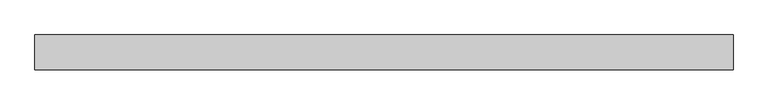
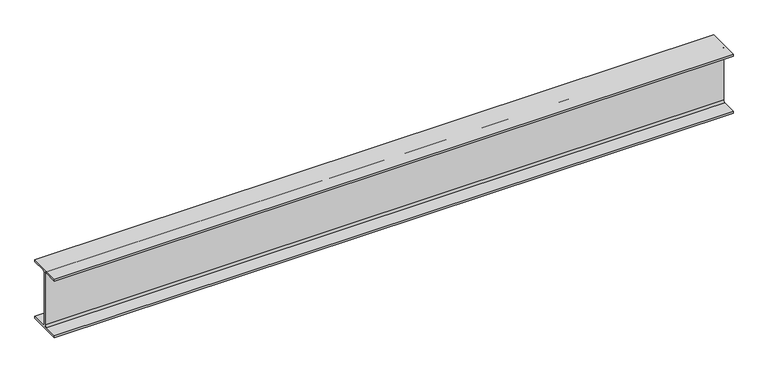
"""IFC4 building model written with IfcOpenShell, lengths in millimetres: beam geometry, Old_Steel Beam_H-KSD3502 : H_SB_ASB_H-200×200x8x12."""

import ifcopenshell
import ifcopenshell.guid

model = None  # the IFC model being written
_history = None  # IfcOwnerHistory: only IFC2X3 demands one
_inside = {}  # id of a spatial element -> (the spatial element, [elements in it])
_under = {}  # id of a project, library or spatial element -> (it, [spatial elements below it])
_declared = {}  # id of a project -> (the project, [libraries it declares])
_typed = {}  # id of a type object -> (the type object, [elements of that type])
_made_of = {}  # id of a material, layer set ... -> (it, [elements and type objects made of it])


def new_model(schema):
    """Start an empty IFC model of exactly this schema.

    Asked for "IFC4X3", IfcOpenShell would pick the latest addendum, in which some entities
    have other attributes; the version numbers below select the first issue.
    IFC2X3 requires an IfcOwnerHistory on every rooted entity: one is made here for all.
    """
    global model, _history
    if schema == "IFC4X3":
        model = ifcopenshell.file(schema_version=(4, 3, 0, 0))
    else:
        model = ifcopenshell.file(schema=schema)
    _inside.clear()
    _under.clear()
    _declared.clear()
    _typed.clear()
    _made_of.clear()
    _history = None
    if model.schema == "IFC2X3":
        org = make("IfcOrganization", Name="unknown")
        user = make(
            "IfcPersonAndOrganization",
            ThePerson=make("IfcPerson", FamilyName="unknown"),
            TheOrganization=org,
        )
        app = make(
            "IfcApplication",
            ApplicationDeveloper=org,
            Version="unknown",
            ApplicationFullName="unknown",
            ApplicationIdentifier="unknown",
        )
        _history = make(
            "IfcOwnerHistory",
            OwningUser=user,
            OwningApplication=app,
            ChangeAction="ADDED",
            CreationDate=0,
        )
    return model


def make(cls, **values):
    """One entity of the class cls with the attributes given. An attribute that is None is left unset."""
    return model.create_entity(
        cls, **{name: value for name, value in values.items() if value is not None}
    )


def rooted(cls, **values):
    """An entity with a GlobalId (a new one), such as an element, a storey or a relation."""
    return make(cls, GlobalId=ifcopenshell.guid.new(), OwnerHistory=_history, **values)


def si_unit(unit_type, name, prefix=None):
    """IfcSIUnit, for example si_unit("LENGTHUNIT", "METRE", prefix="MILLI")."""
    return make("IfcSIUnit", UnitType=unit_type, Prefix=prefix, Name=name)


def assignment(units):
    """IfcUnitAssignment: the units of a project."""
    return None if units is None else make("IfcUnitAssignment", Units=units)


def point(xyz):
    """IfcCartesianPoint."""
    return None if xyz is None else make("IfcCartesianPoint", Coordinates=xyz)


def direction(xyz):
    """IfcDirection."""
    return None if xyz is None else make("IfcDirection", DirectionRatios=xyz)


def frame(location, z_axis=None, x_axis=None):
    """IfcAxis2Placement3D, a coordinate frame: its origin and axes. An axis left out is left unset."""
    return make(
        "IfcAxis2Placement3D",
        Location=point(location),
        Axis=direction(z_axis),
        RefDirection=direction(x_axis),
    )


def frame_2d(location, x_axis=None):
    """IfcAxis2Placement2D, a coordinate frame in the plane: its origin and x axis."""
    return make(
        "IfcAxis2Placement2D", Location=point(location), RefDirection=direction(x_axis)
    )


def origin():
    """The frame at (0, 0, 0) with its axes left unset."""
    return frame((0.0, 0.0, 0.0))


def place(relative_to, where):
    """IfcLocalPlacement: puts the frame where relative to a parent placement (None: the world)."""
    return make(
        "IfcLocalPlacement", PlacementRelTo=relative_to, RelativePlacement=where
    )


def context(
    kind, dimensions, precision=None, world=None, true_north=None, identifier=None
):
    """IfcGeometricRepresentationContext, for example the 3D "Model" context."""
    return make(
        "IfcGeometricRepresentationContext",
        ContextIdentifier=identifier,
        ContextType=kind,
        CoordinateSpaceDimension=dimensions,
        Precision=precision,
        WorldCoordinateSystem=world,
        TrueNorth=true_north,
    )


def project(units=None, contexts=None):
    """IfcProject with its units and contexts."""
    return rooted(
        "IfcProject",
        Name="project",
        RepresentationContexts=contexts,
        UnitsInContext=assignment(units),
    )


def spatial(cls, under=None, at=None, **own):
    """A site, building, storey or space (cls), placed at a placement, below another one or the project."""
    s = rooted(cls, ObjectPlacement=at, **own)
    if under is not None:
        _under.setdefault(under.id(), (under, []))[1].append(s)
    return s


def polyline(points):
    """IfcPolyline through the points."""
    return make("IfcPolyline", Points=[point(p) for p in points])


def circle_curve(where, radius):
    """IfcCircle in the frame where."""
    return make("IfcCircle", Position=where, Radius=radius)


def trimmed(basis, trim1, trim2, sense, master):
    """IfcTrimmedCurve: the piece of a basis curve between two trims."""
    return make(
        "IfcTrimmedCurve",
        BasisCurve=basis,
        Trim1=trim1,
        Trim2=trim2,
        SenseAgreement=sense,
        MasterRepresentation=master,
    )


def segment(curve, same_sense, transition):
    """IfcCompositeCurveSegment."""
    return make(
        "IfcCompositeCurveSegment",
        Transition=transition,
        SameSense=same_sense,
        ParentCurve=curve,
    )


def composite_curve(segments, self_intersect=None):
    """IfcCompositeCurve: segments joined end to end."""
    return make("IfcCompositeCurve", Segments=segments, SelfIntersect=self_intersect)


def outline(outer, holes=None, kind="AREA"):
    """IfcArbitraryClosedProfileDef: a profile drawn as a closed curve; with holes, ...WithVoids."""
    if holes is None:
        return make("IfcArbitraryClosedProfileDef", ProfileType=kind, OuterCurve=outer)
    return make(
        "IfcArbitraryProfileDefWithVoids",
        ProfileType=kind,
        OuterCurve=outer,
        InnerCurves=holes,
    )


def extrude(swept, where, along, depth):
    """IfcExtrudedAreaSolid: the profile swept, set in the frame where, extruded along a direction by depth."""
    return make(
        "IfcExtrudedAreaSolid",
        SweptArea=swept,
        Position=where,
        ExtrudedDirection=direction(along),
        Depth=depth,
    )


def shape(context_of_items, identifier, shape_type, items):
    """IfcShapeRepresentation: the items that make up one representation, for example the "Body"."""
    return make(
        "IfcShapeRepresentation",
        ContextOfItems=context_of_items,
        RepresentationIdentifier=identifier,
        RepresentationType=shape_type,
        Items=items,
    )


def source(mapping_origin, context_of_items, identifier, shape_type, items):
    """IfcRepresentationMap: a shape defined once, which mapped items show again and again."""
    return make(
        "IfcRepresentationMap",
        MappingOrigin=mapping_origin,
        MappedRepresentation=shape(context_of_items, identifier, shape_type, items),
    )


def transform(
    local_origin,
    x_axis=None,
    y_axis=None,
    z_axis=None,
    scale=None,
    scale2=None,
    scale3=None,
    uniform=True,
):
    """IfcCartesianTransformationOperator3D, or its non-uniform kind. x_axis, y_axis, z_axis: its Axis1, 2, 3."""
    if uniform:
        return make(
            "IfcCartesianTransformationOperator3D",
            Axis1=direction(x_axis),
            Axis2=direction(y_axis),
            LocalOrigin=point(local_origin),
            Scale=scale,
            Axis3=direction(z_axis),
        )
    return make(
        "IfcCartesianTransformationOperator3DnonUniform",
        Axis1=direction(x_axis),
        Axis2=direction(y_axis),
        LocalOrigin=point(local_origin),
        Scale=scale,
        Axis3=direction(z_axis),
        Scale2=scale2,
        Scale3=scale3,
    )


def mapped(mapping_source, mapping_target):
    """IfcMappedItem: shows the shape of a source again, moved by a transform."""
    return make(
        "IfcMappedItem", MappingSource=mapping_source, MappingTarget=mapping_target
    )


def made_of(thing, what):
    """Note that an element or type object is made of a material, layer set ...; save() writes the relation."""
    if what is not None:
        _made_of.setdefault(what.id(), (what, []))[1].append(thing)
    return thing


def element(
    cls,
    number,
    at=None,
    inside=None,
    cuts=None,
    type_object=None,
    material=None,
    context=None,
    identifier="Body",
    shape_type=None,
    held_by="IfcProductDefinitionShape",
    body=None,
    shapes=None,
    **own,
):
    """One element of the class cls, such as IfcWall. Its Tag is "e" and its number.

    at: its placement. inside: the storey or other place that contains it. cuts: it is an
    opening in that element (IfcRelVoidsElement). A single representation is given by context,
    identifier, shape_type and body (its items); several are given by shapes. held_by: the class
    of the entity that holds the representations. save() writes the other relations.
    """
    e = rooted(cls, Tag="e%d" % number, ObjectPlacement=at, **own)
    if body is not None:
        shapes = [shape(context, identifier, shape_type, body)]
    if shapes is not None:
        e.Representation = make(held_by, Representations=shapes)
    if inside is not None:
        _inside.setdefault(inside.id(), (inside, []))[1].append(e)
    if cuts is not None:
        rooted(
            "IfcRelVoidsElement", RelatingBuildingElement=cuts, RelatedOpeningElement=e
        )
    if type_object is not None:
        _typed.setdefault(type_object.id(), (type_object, []))[1].append(e)
    return made_of(e, material)


def aggregate(whole, parts):
    """IfcRelAggregates: a whole, such as a stair, and the parts it consists of."""
    return rooted("IfcRelAggregates", RelatingObject=whole, RelatedObjects=parts)


def save(model, path):
    """Write the relations noted so far, then the file.

    IfcRelAggregates (storeys below a building ...), IfcRelContainedInSpatialStructure (elements
    in a storey), IfcRelDefinesByType, IfcRelAssociatesMaterial and IfcRelDeclares: one each for
    every whole, place, type object, material and project.
    """
    for whole, parts in _under.values():
        aggregate(whole, parts)
    for where, things in _inside.values():
        rooted(
            "IfcRelContainedInSpatialStructure",
            RelatedElements=things,
            RelatingStructure=where,
        )
    for kind, things in _typed.values():
        rooted("IfcRelDefinesByType", RelatedObjects=things, RelatingType=kind)
    for what, things in _made_of.values():
        rooted("IfcRelAssociatesMaterial", RelatedObjects=things, RelatingMaterial=what)
    for by, libraries in _declared.values():
        rooted("IfcRelDeclares", RelatingContext=by, RelatedDefinitions=libraries)
    model.write(path)


def beam_5e19d841(model_context):
    return source(origin(), model_context, "Body", "SweptSolid", [
        extrude(outline(composite_curve([segment(polyline([(82.5, -141.5), (82.5, -151.7), (-82.5, -151.7), (-82.5, -141.5), (-11.9, -141.5)]), True, "CONTINUOUS"), segment(trimmed(circle_curve(frame_2d((-11.9, -132.6)), 8.9), [point((-11.9, -141.5))], [point((-3.0, -132.6))], True, "CARTESIAN"), True, "CONTINUOUS"), segment(polyline([(-3.0, -132.6), (-3.0, 132.6)]), True, "CONTINUOUS"), segment(trimmed(circle_curve(frame_2d((-11.9, 132.6)), 8.9), [point((-3.0, 132.6))], [point((-11.9, 141.5))], True, "CARTESIAN"), True, "CONTINUOUS"), segment(polyline([(-11.9, 141.5), (-82.5, 141.5), (-82.5, 151.7), (82.5, 151.7), (82.5, 141.5), (11.9, 141.5)]), True, "CONTINUOUS"), segment(trimmed(circle_curve(frame_2d((11.9, 132.6)), 8.9), [point((11.9, 141.5))], [point((3.0, 132.6))], True, "CARTESIAN"), True, "CONTINUOUS"), segment(polyline([(3.0, 132.6), (3.0, -132.6)]), True, "CONTINUOUS"), segment(trimmed(circle_curve(frame_2d((11.9, -132.6)), 8.9), [point((3.0, -132.6))], [point((11.9, -141.5))], True, "CARTESIAN"), True, "CONTINUOUS"), segment(polyline([(11.9, -141.5), (82.5, -141.5)]), True, "CONTINUOUS")], self_intersect=False)), frame((-1721.7329802, 0.0, 0.0), z_axis=(1.0, 0.0, 0.0), x_axis=(0.0, 1.0, 0.0)), (0.0, 0.0, 1.0), 3316.0486402),
    ])


if __name__ == "__main__":
    model = new_model("IFC4")
    model_context = context("Model", 3, world=origin())
    ifc_project = project(units=[si_unit("LENGTHUNIT", "METRE", prefix="MILLI")], contexts=[model_context])
    site = spatial("IfcSite", under=ifc_project)
    building = spatial("IfcBuilding", under=site)
    placement = place(None, origin())
    beam_shape = beam_5e19d841(model_context)
    element("IfcBeam", 1, ObjectType="Old_Steel Beam_H-KSD3502 : H_SB_ASB_H-200×200x8x12", at=placement, inside=building, context=model_context, shape_type="MappedRepresentation", body=[
        mapped(beam_shape, transform((0.0, 0.0, 0.0), x_axis=(1.0, 0.0, 0.0), y_axis=(0.0, 1.0, 0.0), z_axis=(0.0, 0.0, 1.0))),
    ])
    save(model, "model.ifc")

# Revit data of these elements
# Type "Old_Steel Beam_H-KSD3502 : H_SB_ASB_H-200×200x8x12"
#   Width = 20.0 cm
#   Web Thickness = 0.8 cm
#   Web Fillet = 1.3 cm
#   Warping Constant = 141376.0 cm⁶
#   Torsional Moment of Inertia = 26.2485 cm⁴
#   Torsional Modulus = 1.0 cm³
#   Section Area = 63.53 cm²
#   Plastic Modulus weak axis = 244.0 cm³
#   Plastic Modulus strong axis = 525.0 cm³
#   Perimeter = 1.16 m²/m
#   Nominal Weight = 49.90 kgf/m
#   Moment of Inertia weak axis = 1600.00 cm⁴
#   Moment of Inertia strong axis = 4720.00 cm⁴
#   Height = 20.0 cm
#   Flange Thickness = 1.2 cm
#   Elastic Modulus weak axis = 160.0 cm³
#   Elastic Modulus strong axis = 472.0 cm³
#   Centroid Vertical = 10.0 cm
#   Centroid Horizontal = 10.0 cm
#   Length [instance default] = 1.5240 m
#   Structural Material [instance default] = Steel, 45-345
#   Assembly Code = ""
# Element 1 (IfcBeam, "Old_Steel Beam_H-KSD3502 : H_SB_ASB_H-200×200x8x12")
#   Structural Material = none
# Materials
#   "Steel, 45-345": class "Metal", colour RGB 189 187 185, transparency 0, Description = "Steel 345 MPa", Cost = 0
